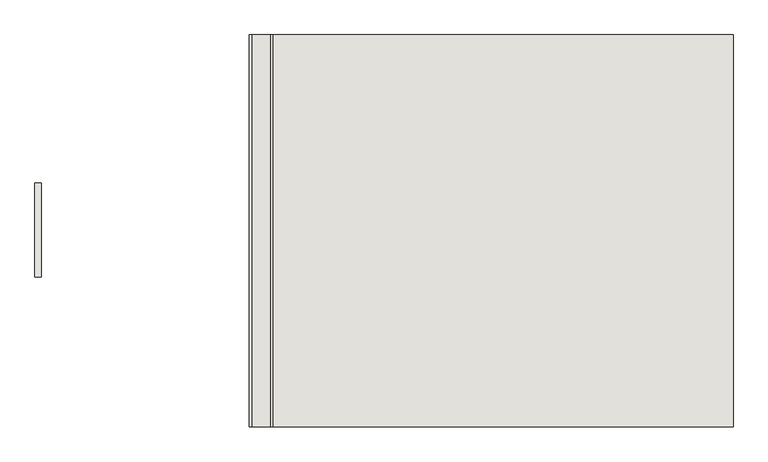
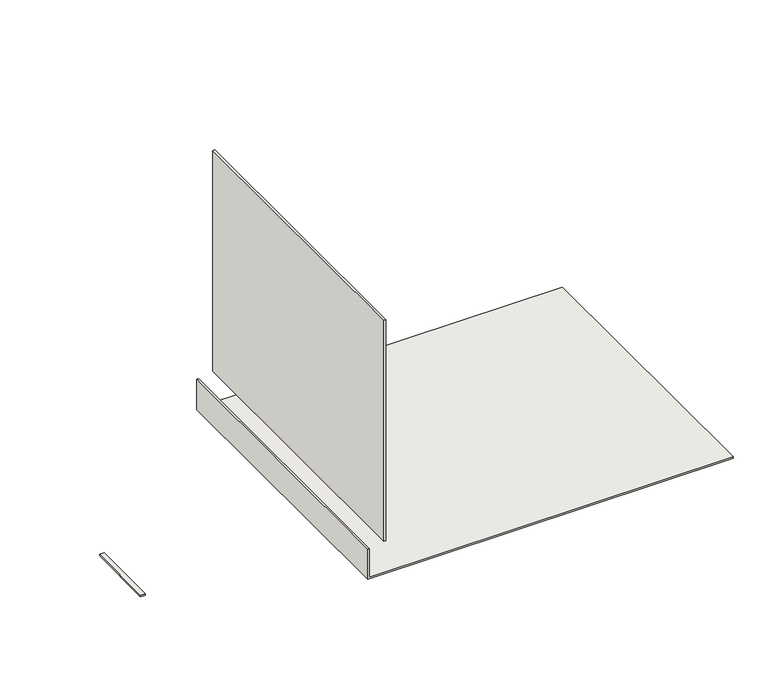
"""IFC4 building model written with IfcOpenShell, lengths in millimetres: wall geometry."""

from ifc_helpers import new_model, si_unit, frame, origin, place, context, project, spatial, polyline, outline, extrude, source, transform, mapped, element, save


def wall_5e231985(model_context):
    return source(origin(), model_context, "Body", "SweptSolid", [
        extrude(outline(polyline([(18072.8870052, -2319.6634634), (18028.2100968, -2319.6634634), (18028.2100968, -1633.8634634), (18072.8870052, -1633.8634634), (18072.8870052, -2319.6634634)])), frame((0.0, 0.0, 2181.225), z_axis=(0.0, 0.0, 1.0), x_axis=(1.0, 0.0, 0.0)), (0.0, 0.0, 1.0), 15.875),
        extrude(outline(polyline([(19765.1620052, -3415.0384634), (19749.2870052, -3415.0384634), (19749.2870052, -552.3178244), (19765.1620052, -552.3178244), (19765.1620052, -3415.0384634)])), frame((0.0, 0.0, 2809.875), z_axis=(0.0, 0.0, 1.0), x_axis=(1.0, 0.0, 0.0)), (0.0, 0.0, 1.0), 2255.9278105),
        extrude(outline(polyline([(2473.325, 19593.7120052), (2473.325, 23124.3120052), (2489.2, 23124.3120052), (2489.2, 19609.5870052), (2781.3, 19609.5870052), (2781.3, 19593.7120052), (2473.325, 19593.7120052)])), frame((0.0, -3415.0384634, 0.0), z_axis=(0.0, 1.0, 0.0), x_axis=(0.0, 0.0, 1.0)), (0.0, 0.0, 1.0), 2862.7206389),
    ])


if __name__ == "__main__":
    model = new_model("IFC4")
    model_context = context("Model", 3, world=origin())
    ifc_project = project(units=[si_unit("LENGTHUNIT", "METRE", prefix="MILLI")], contexts=[model_context])
    site = spatial("IfcSite", under=ifc_project)
    building = spatial("IfcBuilding", under=site)
    placement = place(None, origin())
    wall_shape = wall_5e231985(model_context)
    element("IfcWall", 1, ObjectType="5/8\" GYP. T.B.D. - PAINTED : 5/8\" GYP. T.B.D. - PAINTED", at=placement, inside=building, context=model_context, shape_type="MappedRepresentation", body=[
        mapped(wall_shape, transform((0.0, 0.0, 0.0), x_axis=(1.0, 0.0, 0.0), y_axis=(0.0, 1.0, 0.0), z_axis=(0.0, 0.0, 1.0))),
    ])
    save(model, "model.ifc")

# Revit data of these elements
# Element 1 (IfcWall, "5/8\" GYP. T.B.D. - PAINTED : 5/8\" GYP. T.B.D. - PAINTED")
#   Materials on its faces: "5/8\" GYP. BD - PAINTED"
# Materials
#   "5/8\" GYP. BD - PAINTED": class "Generic", colour RGB 255 255 255, transparency 0, Description = "Gypsum Wall Board", Cost = 0
